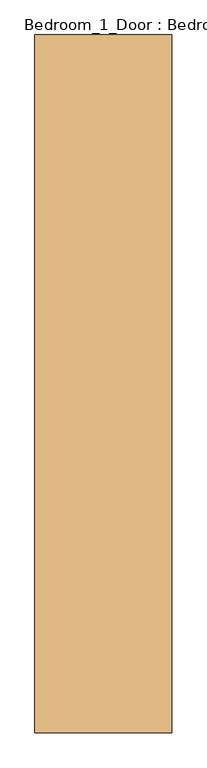
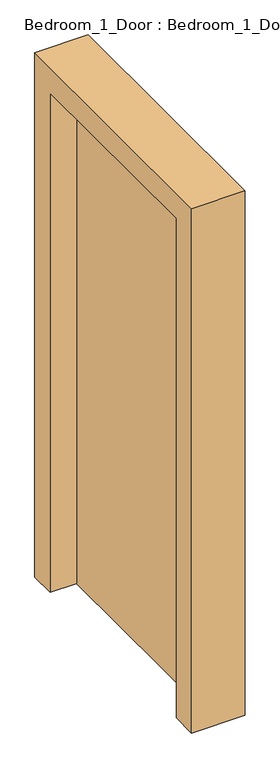
"""IFC4 building model written with IfcOpenShell, lengths in millimetres: door geometry, Bedroom_1_Door : Bedroom_1_Door."""

from ifc_helpers import new_model, si_unit, frame, origin, place, context, project, spatial, polyline, outline, extrude, source, transform, mapped, element, save


def bedroom_1_door_bedroom_1_door_f4a16035(model_context):
    return source(origin(), model_context, "Body", "SweptSolid", [
        extrude(outline(polyline([(2000.0, 3675.0), (2000.0, 4495.0), (2100.0, 4495.0), (2100.0, 3675.0), (2000.0, 3675.0)])), frame((0.0, 0.0, 250.0), z_axis=(0.0, 0.0, 1.0), x_axis=(1.0, 0.0, 0.0)), (0.0, 0.0, 1.0), 1980.0),
        extrude(outline(polyline([(4595.0, 250.0), (4495.0, 250.0), (4495.0, 2230.0), (3675.0, 2230.0), (3675.0, 250.0), (3575.0, 250.0), (3575.0, 2330.0), (4595.0, 2330.0), (4595.0, 250.0)])), frame((1900.0, 0.0, 0.0), z_axis=(1.0, 0.0, 0.0), x_axis=(0.0, 1.0, 0.0)), (0.0, 0.0, 1.0), 200.0),
    ])


if __name__ == "__main__":
    model = new_model("IFC4")
    model_context = context("Model", 3, world=origin())
    ifc_project = project(units=[si_unit("LENGTHUNIT", "METRE", prefix="MILLI")], contexts=[model_context])
    site = spatial("IfcSite", under=ifc_project)
    building = spatial("IfcBuilding", under=site)
    placement = place(None, origin())
    bedroom_1_door_bedroom_1_door_shape = bedroom_1_door_bedroom_1_door_f4a16035(model_context)
    element("IfcDoor", 1, ObjectType="Bedroom_1_Door : Bedroom_1_Door", at=placement, inside=building, context=model_context, shape_type="MappedRepresentation", body=[
        mapped(bedroom_1_door_bedroom_1_door_shape, transform((0.0, 0.0, 0.0), x_axis=(1.0, 0.0, 0.0), y_axis=(0.0, 1.0, 0.0), z_axis=(0.0, 0.0, 1.0))),
    ])
    save(model, "model.ifc")

# Revit data of these elements
# Type "Bedroom_1_Door : Bedroom_1_Door"
#   Type Mark = "48"
#   NameOverride = "Bedroom_1_Door"
# Element 1 (IfcDoor, "Bedroom_1_Door : Bedroom_1_Door")
#   Materials on its faces: "IfcSurfaceStyle #392"
# Materials
#   "IfcSurfaceStyle #392": class "Unassigned", colour RGB 204 204 204, transparency 0
